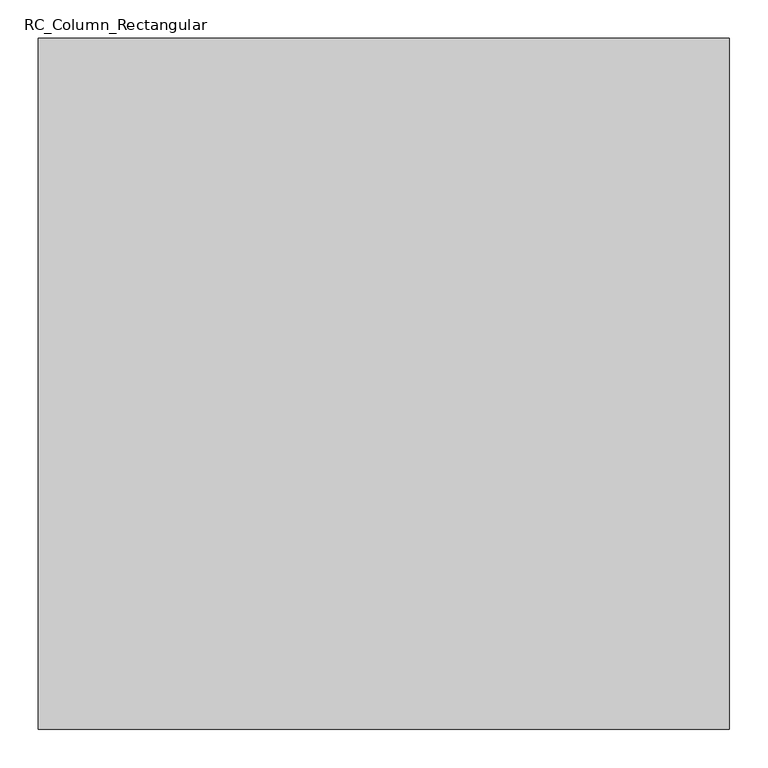
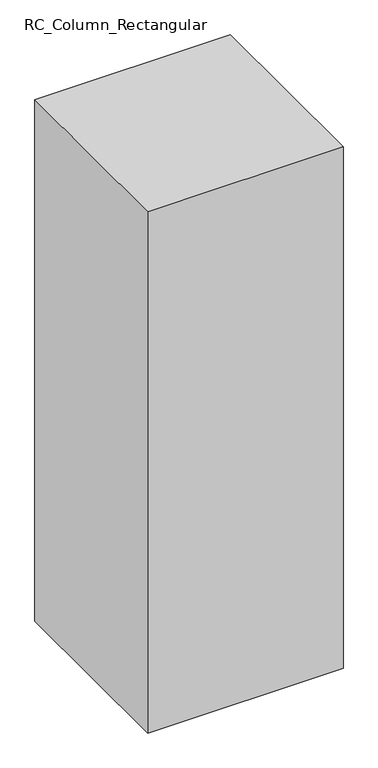
"""IFC4 building model written with IfcOpenShell, lengths in millimetres: column geometry, RC_Column_Rectangular : H_SC_AR_S15_AG Column_900x900_C2."""

import ifcopenshell
import ifcopenshell.guid

model = None  # the IFC model being written
_history = None  # IfcOwnerHistory: only IFC2X3 demands one
_inside = {}  # id of a spatial element -> (the spatial element, [elements in it])
_under = {}  # id of a project, library or spatial element -> (it, [spatial elements below it])
_declared = {}  # id of a project -> (the project, [libraries it declares])
_typed = {}  # id of a type object -> (the type object, [elements of that type])
_made_of = {}  # id of a material, layer set ... -> (it, [elements and type objects made of it])


def new_model(schema):
    """Start an empty IFC model of exactly this schema.

    Asked for "IFC4X3", IfcOpenShell would pick the latest addendum, in which some entities
    have other attributes; the version numbers below select the first issue.
    IFC2X3 requires an IfcOwnerHistory on every rooted entity: one is made here for all.
    """
    global model, _history
    if schema == "IFC4X3":
        model = ifcopenshell.file(schema_version=(4, 3, 0, 0))
    else:
        model = ifcopenshell.file(schema=schema)
    _inside.clear()
    _under.clear()
    _declared.clear()
    _typed.clear()
    _made_of.clear()
    _history = None
    if model.schema == "IFC2X3":
        org = make("IfcOrganization", Name="unknown")
        user = make(
            "IfcPersonAndOrganization",
            ThePerson=make("IfcPerson", FamilyName="unknown"),
            TheOrganization=org,
        )
        app = make(
            "IfcApplication",
            ApplicationDeveloper=org,
            Version="unknown",
            ApplicationFullName="unknown",
            ApplicationIdentifier="unknown",
        )
        _history = make(
            "IfcOwnerHistory",
            OwningUser=user,
            OwningApplication=app,
            ChangeAction="ADDED",
            CreationDate=0,
        )
    return model


def make(cls, **values):
    """One entity of the class cls with the attributes given. An attribute that is None is left unset."""
    return model.create_entity(
        cls, **{name: value for name, value in values.items() if value is not None}
    )


def rooted(cls, **values):
    """An entity with a GlobalId (a new one), such as an element, a storey or a relation."""
    return make(cls, GlobalId=ifcopenshell.guid.new(), OwnerHistory=_history, **values)


def si_unit(unit_type, name, prefix=None):
    """IfcSIUnit, for example si_unit("LENGTHUNIT", "METRE", prefix="MILLI")."""
    return make("IfcSIUnit", UnitType=unit_type, Prefix=prefix, Name=name)


def assignment(units):
    """IfcUnitAssignment: the units of a project."""
    return None if units is None else make("IfcUnitAssignment", Units=units)


def point(xyz):
    """IfcCartesianPoint."""
    return None if xyz is None else make("IfcCartesianPoint", Coordinates=xyz)


def direction(xyz):
    """IfcDirection."""
    return None if xyz is None else make("IfcDirection", DirectionRatios=xyz)


def frame(location, z_axis=None, x_axis=None):
    """IfcAxis2Placement3D, a coordinate frame: its origin and axes. An axis left out is left unset."""
    return make(
        "IfcAxis2Placement3D",
        Location=point(location),
        Axis=direction(z_axis),
        RefDirection=direction(x_axis),
    )


def origin():
    """The frame at (0, 0, 0) with its axes left unset."""
    return frame((0.0, 0.0, 0.0))


def place(relative_to, where):
    """IfcLocalPlacement: puts the frame where relative to a parent placement (None: the world)."""
    return make(
        "IfcLocalPlacement", PlacementRelTo=relative_to, RelativePlacement=where
    )


def context(
    kind, dimensions, precision=None, world=None, true_north=None, identifier=None
):
    """IfcGeometricRepresentationContext, for example the 3D "Model" context."""
    return make(
        "IfcGeometricRepresentationContext",
        ContextIdentifier=identifier,
        ContextType=kind,
        CoordinateSpaceDimension=dimensions,
        Precision=precision,
        WorldCoordinateSystem=world,
        TrueNorth=true_north,
    )


def project(units=None, contexts=None):
    """IfcProject with its units and contexts."""
    return rooted(
        "IfcProject",
        Name="project",
        RepresentationContexts=contexts,
        UnitsInContext=assignment(units),
    )


def spatial(cls, under=None, at=None, **own):
    """A site, building, storey or space (cls), placed at a placement, below another one or the project."""
    s = rooted(cls, ObjectPlacement=at, **own)
    if under is not None:
        _under.setdefault(under.id(), (under, []))[1].append(s)
    return s


def polyline(points):
    """IfcPolyline through the points."""
    return make("IfcPolyline", Points=[point(p) for p in points])


def outline(outer, holes=None, kind="AREA"):
    """IfcArbitraryClosedProfileDef: a profile drawn as a closed curve; with holes, ...WithVoids."""
    if holes is None:
        return make("IfcArbitraryClosedProfileDef", ProfileType=kind, OuterCurve=outer)
    return make(
        "IfcArbitraryProfileDefWithVoids",
        ProfileType=kind,
        OuterCurve=outer,
        InnerCurves=holes,
    )


def extrude(swept, where, along, depth):
    """IfcExtrudedAreaSolid: the profile swept, set in the frame where, extruded along a direction by depth."""
    return make(
        "IfcExtrudedAreaSolid",
        SweptArea=swept,
        Position=where,
        ExtrudedDirection=direction(along),
        Depth=depth,
    )


def shape(context_of_items, identifier, shape_type, items):
    """IfcShapeRepresentation: the items that make up one representation, for example the "Body"."""
    return make(
        "IfcShapeRepresentation",
        ContextOfItems=context_of_items,
        RepresentationIdentifier=identifier,
        RepresentationType=shape_type,
        Items=items,
    )


def source(mapping_origin, context_of_items, identifier, shape_type, items):
    """IfcRepresentationMap: a shape defined once, which mapped items show again and again."""
    return make(
        "IfcRepresentationMap",
        MappingOrigin=mapping_origin,
        MappedRepresentation=shape(context_of_items, identifier, shape_type, items),
    )


def transform(
    local_origin,
    x_axis=None,
    y_axis=None,
    z_axis=None,
    scale=None,
    scale2=None,
    scale3=None,
    uniform=True,
):
    """IfcCartesianTransformationOperator3D, or its non-uniform kind. x_axis, y_axis, z_axis: its Axis1, 2, 3."""
    if uniform:
        return make(
            "IfcCartesianTransformationOperator3D",
            Axis1=direction(x_axis),
            Axis2=direction(y_axis),
            LocalOrigin=point(local_origin),
            Scale=scale,
            Axis3=direction(z_axis),
        )
    return make(
        "IfcCartesianTransformationOperator3DnonUniform",
        Axis1=direction(x_axis),
        Axis2=direction(y_axis),
        LocalOrigin=point(local_origin),
        Scale=scale,
        Axis3=direction(z_axis),
        Scale2=scale2,
        Scale3=scale3,
    )


def mapped(mapping_source, mapping_target):
    """IfcMappedItem: shows the shape of a source again, moved by a transform."""
    return make(
        "IfcMappedItem", MappingSource=mapping_source, MappingTarget=mapping_target
    )


def made_of(thing, what):
    """Note that an element or type object is made of a material, layer set ...; save() writes the relation."""
    if what is not None:
        _made_of.setdefault(what.id(), (what, []))[1].append(thing)
    return thing


def element(
    cls,
    number,
    at=None,
    inside=None,
    cuts=None,
    type_object=None,
    material=None,
    context=None,
    identifier="Body",
    shape_type=None,
    held_by="IfcProductDefinitionShape",
    body=None,
    shapes=None,
    **own,
):
    """One element of the class cls, such as IfcWall. Its Tag is "e" and its number.

    at: its placement. inside: the storey or other place that contains it. cuts: it is an
    opening in that element (IfcRelVoidsElement). A single representation is given by context,
    identifier, shape_type and body (its items); several are given by shapes. held_by: the class
    of the entity that holds the representations. save() writes the other relations.
    """
    e = rooted(cls, Tag="e%d" % number, ObjectPlacement=at, **own)
    if body is not None:
        shapes = [shape(context, identifier, shape_type, body)]
    if shapes is not None:
        e.Representation = make(held_by, Representations=shapes)
    if inside is not None:
        _inside.setdefault(inside.id(), (inside, []))[1].append(e)
    if cuts is not None:
        rooted(
            "IfcRelVoidsElement", RelatingBuildingElement=cuts, RelatedOpeningElement=e
        )
    if type_object is not None:
        _typed.setdefault(type_object.id(), (type_object, []))[1].append(e)
    return made_of(e, material)


def aggregate(whole, parts):
    """IfcRelAggregates: a whole, such as a stair, and the parts it consists of."""
    return rooted("IfcRelAggregates", RelatingObject=whole, RelatedObjects=parts)


def save(model, path):
    """Write the relations noted so far, then the file.

    IfcRelAggregates (storeys below a building ...), IfcRelContainedInSpatialStructure (elements
    in a storey), IfcRelDefinesByType, IfcRelAssociatesMaterial and IfcRelDeclares: one each for
    every whole, place, type object, material and project.
    """
    for whole, parts in _under.values():
        aggregate(whole, parts)
    for where, things in _inside.values():
        rooted(
            "IfcRelContainedInSpatialStructure",
            RelatedElements=things,
            RelatingStructure=where,
        )
    for kind, things in _typed.values():
        rooted("IfcRelDefinesByType", RelatedObjects=things, RelatingType=kind)
    for what, things in _made_of.values():
        rooted("IfcRelAssociatesMaterial", RelatedObjects=things, RelatingMaterial=what)
    for by, libraries in _declared.values():
        rooted("IfcRelDeclares", RelatingContext=by, RelatedDefinitions=libraries)
    model.write(path)


def rc_column_rectangular_84820dcc(model_context):
    return source(origin(), model_context, "Body", "SweptSolid", [
        extrude(outline(polyline([(450.0, 450.0), (450.0, -450.0), (-450.0, -450.0), (-450.0, 450.0), (450.0, 450.0)])), frame((0.0, 0.0, 4799.9618634), z_axis=(0.0, 0.0, 1.0), x_axis=(1.0, 0.0, 0.0)), (0.0, 0.0, 1.0), 2540.0381366),
    ])


if __name__ == "__main__":
    model = new_model("IFC4")
    model_context = context("Model", 3, world=origin())
    ifc_project = project(units=[si_unit("LENGTHUNIT", "METRE", prefix="MILLI")], contexts=[model_context])
    site = spatial("IfcSite", under=ifc_project)
    building = spatial("IfcBuilding", under=site)
    placement = place(None, origin())
    rc_column_rectangular_shape = rc_column_rectangular_84820dcc(model_context)
    element("IfcColumn", 1, ObjectType="RC_Column_Rectangular : H_SC_AR_S15_AG Column_900x900_C2", at=placement, inside=building, context=model_context, shape_type="MappedRepresentation", body=[
        mapped(rc_column_rectangular_shape, transform((0.0, 0.0, 0.0), x_axis=(1.0, 0.0, 0.0), y_axis=(0.0, 1.0, 0.0), z_axis=(0.0, 0.0, 1.0))),
    ])
    save(model, "model.ifc")

# Revit data of these elements
# Type "RC_Column_Rectangular : H_SC_AR_S15_AG Column_900x900_C2"
#   Width = 900 mm
#   Length = 900 mm
#   hec_material3 [instance default] = none
#   hec_material2 [instance default] = none
#   hec_material1 [instance default] = none
#   Structural Material [instance default] = none
#   Description = (empty or 0)
# Element 1 (IfcColumn, "RC_Column_Rectangular : H_SC_AR_S15_AG Column_900x900_C2")
#   Structural Material = Concrete_f'c=28MPa(Cylender)
#   Materials on its faces: "Concrete_f'c=28MPa(Cylender)"
# Materials
#   "Concrete_f'c=28MPa(Cylender)": class "Concrete", colour RGB 176 176 176, transparency 0, Description = "Reinf. Conc.", Cost = 0, Image = Concrete.Cast-In-Place.Flat.Polished.Grey.jpg
